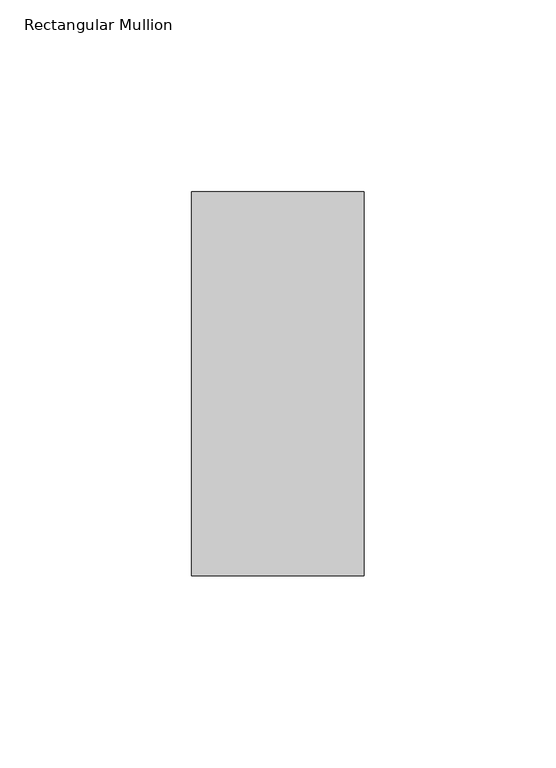
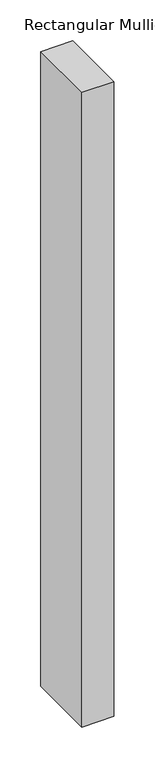
"""IFC4 building model written with IfcOpenShell, lengths in millimetres: member geometry, Rectangular Mullion : 알루미늄_Rectangular Cap_100 x 45."""

from ifc_helpers import new_model, si_unit, frame, origin, place, context, project, spatial, polyline, outline, extrude, source, transform, mapped, element, save


def rectangular_mullion_ca7a66ac(model_context):
    return source(origin(), model_context, "Body", "SweptSolid", [
        extrude(outline(polyline([(22.5, 50.0), (22.5, -50.0), (-22.5, -50.0), (-22.5, 50.0), (22.5, 50.0)])), frame((0.0, 0.0, -945.0), z_axis=(0.0, 0.0, 1.0), x_axis=(1.0, 0.0, 0.0)), (0.0, 0.0, 1.0), 945.0),
    ])


if __name__ == "__main__":
    model = new_model("IFC4")
    model_context = context("Model", 3, world=origin())
    ifc_project = project(units=[si_unit("LENGTHUNIT", "METRE", prefix="MILLI")], contexts=[model_context])
    site = spatial("IfcSite", under=ifc_project)
    building = spatial("IfcBuilding", under=site)
    placement = place(None, origin())
    rectangular_mullion_shape = rectangular_mullion_ca7a66ac(model_context)
    element("IfcMember", 1, ObjectType="Rectangular Mullion : 알루미늄_Rectangular Cap_100 x 45", at=placement, inside=building, context=model_context, shape_type="MappedRepresentation", body=[
        mapped(rectangular_mullion_shape, transform((0.0, 0.0, 0.0), x_axis=(1.0, 0.0, 0.0), y_axis=(0.0, 1.0, 0.0), z_axis=(0.0, 0.0, 1.0))),
    ])
    save(model, "model.ifc")

# Revit data of these elements
# Type "Rectangular Mullion : 알루미늄_Rectangular Cap_100 x 45"
#   built-in parameter 1007304 = 0.328084 (stored number, unit not read)
#   built-in parameter 1007301 = 0.0738189 (stored number, unit not read)
#   built-in parameter 1007300 = 0.0738189 (stored number, unit not read)
# Element 1 (IfcMember, "Rectangular Mullion : 알루미늄_Rectangular Cap_100 x 45")
#   Materials on its faces: "00_Metal_Stainless Steel"
# Materials
#   "00_Metal_Stainless Steel": class "Metal", colour RGB 148 148 148, transparency 0, Description = "Steel", Cost = 0
